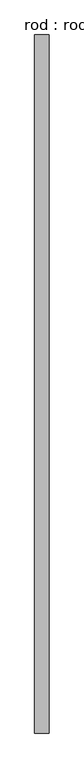
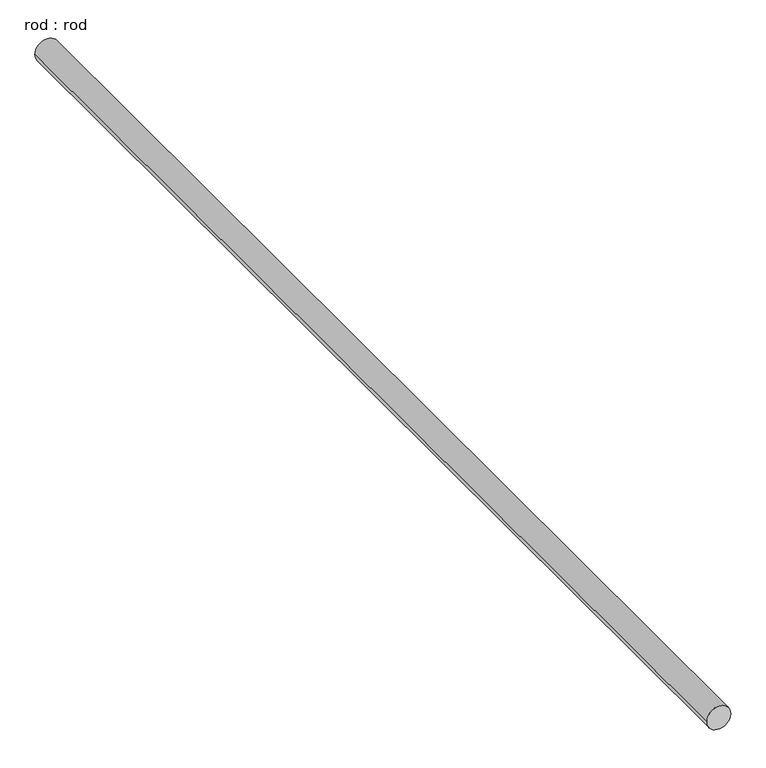
"""IFC4 building model written with IfcOpenShell, lengths in millimetres: proxy geometry, rod : rod."""

import ifcopenshell
import ifcopenshell.guid

model = None  # the IFC model being written
_history = None  # IfcOwnerHistory: only IFC2X3 demands one
_inside = {}  # id of a spatial element -> (the spatial element, [elements in it])
_under = {}  # id of a project, library or spatial element -> (it, [spatial elements below it])
_declared = {}  # id of a project -> (the project, [libraries it declares])
_typed = {}  # id of a type object -> (the type object, [elements of that type])
_made_of = {}  # id of a material, layer set ... -> (it, [elements and type objects made of it])


def new_model(schema):
    """Start an empty IFC model of exactly this schema.

    Asked for "IFC4X3", IfcOpenShell would pick the latest addendum, in which some entities
    have other attributes; the version numbers below select the first issue.
    IFC2X3 requires an IfcOwnerHistory on every rooted entity: one is made here for all.
    """
    global model, _history
    if schema == "IFC4X3":
        model = ifcopenshell.file(schema_version=(4, 3, 0, 0))
    else:
        model = ifcopenshell.file(schema=schema)
    _inside.clear()
    _under.clear()
    _declared.clear()
    _typed.clear()
    _made_of.clear()
    _history = None
    if model.schema == "IFC2X3":
        org = make("IfcOrganization", Name="unknown")
        user = make(
            "IfcPersonAndOrganization",
            ThePerson=make("IfcPerson", FamilyName="unknown"),
            TheOrganization=org,
        )
        app = make(
            "IfcApplication",
            ApplicationDeveloper=org,
            Version="unknown",
            ApplicationFullName="unknown",
            ApplicationIdentifier="unknown",
        )
        _history = make(
            "IfcOwnerHistory",
            OwningUser=user,
            OwningApplication=app,
            ChangeAction="ADDED",
            CreationDate=0,
        )
    return model


def make(cls, **values):
    """One entity of the class cls with the attributes given. An attribute that is None is left unset."""
    return model.create_entity(
        cls, **{name: value for name, value in values.items() if value is not None}
    )


def rooted(cls, **values):
    """An entity with a GlobalId (a new one), such as an element, a storey or a relation."""
    return make(cls, GlobalId=ifcopenshell.guid.new(), OwnerHistory=_history, **values)


def si_unit(unit_type, name, prefix=None):
    """IfcSIUnit, for example si_unit("LENGTHUNIT", "METRE", prefix="MILLI")."""
    return make("IfcSIUnit", UnitType=unit_type, Prefix=prefix, Name=name)


def assignment(units):
    """IfcUnitAssignment: the units of a project."""
    return None if units is None else make("IfcUnitAssignment", Units=units)


def point(xyz):
    """IfcCartesianPoint."""
    return None if xyz is None else make("IfcCartesianPoint", Coordinates=xyz)


def direction(xyz):
    """IfcDirection."""
    return None if xyz is None else make("IfcDirection", DirectionRatios=xyz)


def frame(location, z_axis=None, x_axis=None):
    """IfcAxis2Placement3D, a coordinate frame: its origin and axes. An axis left out is left unset."""
    return make(
        "IfcAxis2Placement3D",
        Location=point(location),
        Axis=direction(z_axis),
        RefDirection=direction(x_axis),
    )


def frame_2d(location, x_axis=None):
    """IfcAxis2Placement2D, a coordinate frame in the plane: its origin and x axis."""
    return make(
        "IfcAxis2Placement2D", Location=point(location), RefDirection=direction(x_axis)
    )


def origin():
    """The frame at (0, 0, 0) with its axes left unset."""
    return frame((0.0, 0.0, 0.0))


def place(relative_to, where):
    """IfcLocalPlacement: puts the frame where relative to a parent placement (None: the world)."""
    return make(
        "IfcLocalPlacement", PlacementRelTo=relative_to, RelativePlacement=where
    )


def context(
    kind, dimensions, precision=None, world=None, true_north=None, identifier=None
):
    """IfcGeometricRepresentationContext, for example the 3D "Model" context."""
    return make(
        "IfcGeometricRepresentationContext",
        ContextIdentifier=identifier,
        ContextType=kind,
        CoordinateSpaceDimension=dimensions,
        Precision=precision,
        WorldCoordinateSystem=world,
        TrueNorth=true_north,
    )


def project(units=None, contexts=None):
    """IfcProject with its units and contexts."""
    return rooted(
        "IfcProject",
        Name="project",
        RepresentationContexts=contexts,
        UnitsInContext=assignment(units),
    )


def spatial(cls, under=None, at=None, **own):
    """A site, building, storey or space (cls), placed at a placement, below another one or the project."""
    s = rooted(cls, ObjectPlacement=at, **own)
    if under is not None:
        _under.setdefault(under.id(), (under, []))[1].append(s)
    return s


def circle_curve(where, radius):
    """IfcCircle in the frame where."""
    return make("IfcCircle", Position=where, Radius=radius)


def trimmed(basis, trim1, trim2, sense, master):
    """IfcTrimmedCurve: the piece of a basis curve between two trims."""
    return make(
        "IfcTrimmedCurve",
        BasisCurve=basis,
        Trim1=trim1,
        Trim2=trim2,
        SenseAgreement=sense,
        MasterRepresentation=master,
    )


def segment(curve, same_sense, transition):
    """IfcCompositeCurveSegment."""
    return make(
        "IfcCompositeCurveSegment",
        Transition=transition,
        SameSense=same_sense,
        ParentCurve=curve,
    )


def composite_curve(segments, self_intersect=None):
    """IfcCompositeCurve: segments joined end to end."""
    return make("IfcCompositeCurve", Segments=segments, SelfIntersect=self_intersect)


def outline(outer, holes=None, kind="AREA"):
    """IfcArbitraryClosedProfileDef: a profile drawn as a closed curve; with holes, ...WithVoids."""
    if holes is None:
        return make("IfcArbitraryClosedProfileDef", ProfileType=kind, OuterCurve=outer)
    return make(
        "IfcArbitraryProfileDefWithVoids",
        ProfileType=kind,
        OuterCurve=outer,
        InnerCurves=holes,
    )


def extrude(swept, where, along, depth):
    """IfcExtrudedAreaSolid: the profile swept, set in the frame where, extruded along a direction by depth."""
    return make(
        "IfcExtrudedAreaSolid",
        SweptArea=swept,
        Position=where,
        ExtrudedDirection=direction(along),
        Depth=depth,
    )


def shape(context_of_items, identifier, shape_type, items):
    """IfcShapeRepresentation: the items that make up one representation, for example the "Body"."""
    return make(
        "IfcShapeRepresentation",
        ContextOfItems=context_of_items,
        RepresentationIdentifier=identifier,
        RepresentationType=shape_type,
        Items=items,
    )


def source(mapping_origin, context_of_items, identifier, shape_type, items):
    """IfcRepresentationMap: a shape defined once, which mapped items show again and again."""
    return make(
        "IfcRepresentationMap",
        MappingOrigin=mapping_origin,
        MappedRepresentation=shape(context_of_items, identifier, shape_type, items),
    )


def transform(
    local_origin,
    x_axis=None,
    y_axis=None,
    z_axis=None,
    scale=None,
    scale2=None,
    scale3=None,
    uniform=True,
):
    """IfcCartesianTransformationOperator3D, or its non-uniform kind. x_axis, y_axis, z_axis: its Axis1, 2, 3."""
    if uniform:
        return make(
            "IfcCartesianTransformationOperator3D",
            Axis1=direction(x_axis),
            Axis2=direction(y_axis),
            LocalOrigin=point(local_origin),
            Scale=scale,
            Axis3=direction(z_axis),
        )
    return make(
        "IfcCartesianTransformationOperator3DnonUniform",
        Axis1=direction(x_axis),
        Axis2=direction(y_axis),
        LocalOrigin=point(local_origin),
        Scale=scale,
        Axis3=direction(z_axis),
        Scale2=scale2,
        Scale3=scale3,
    )


def mapped(mapping_source, mapping_target):
    """IfcMappedItem: shows the shape of a source again, moved by a transform."""
    return make(
        "IfcMappedItem", MappingSource=mapping_source, MappingTarget=mapping_target
    )


def made_of(thing, what):
    """Note that an element or type object is made of a material, layer set ...; save() writes the relation."""
    if what is not None:
        _made_of.setdefault(what.id(), (what, []))[1].append(thing)
    return thing


def element(
    cls,
    number,
    at=None,
    inside=None,
    cuts=None,
    type_object=None,
    material=None,
    context=None,
    identifier="Body",
    shape_type=None,
    held_by="IfcProductDefinitionShape",
    body=None,
    shapes=None,
    **own,
):
    """One element of the class cls, such as IfcWall. Its Tag is "e" and its number.

    at: its placement. inside: the storey or other place that contains it. cuts: it is an
    opening in that element (IfcRelVoidsElement). A single representation is given by context,
    identifier, shape_type and body (its items); several are given by shapes. held_by: the class
    of the entity that holds the representations. save() writes the other relations.
    """
    e = rooted(cls, Tag="e%d" % number, ObjectPlacement=at, **own)
    if body is not None:
        shapes = [shape(context, identifier, shape_type, body)]
    if shapes is not None:
        e.Representation = make(held_by, Representations=shapes)
    if inside is not None:
        _inside.setdefault(inside.id(), (inside, []))[1].append(e)
    if cuts is not None:
        rooted(
            "IfcRelVoidsElement", RelatingBuildingElement=cuts, RelatedOpeningElement=e
        )
    if type_object is not None:
        _typed.setdefault(type_object.id(), (type_object, []))[1].append(e)
    return made_of(e, material)


def aggregate(whole, parts):
    """IfcRelAggregates: a whole, such as a stair, and the parts it consists of."""
    return rooted("IfcRelAggregates", RelatingObject=whole, RelatedObjects=parts)


def save(model, path):
    """Write the relations noted so far, then the file.

    IfcRelAggregates (storeys below a building ...), IfcRelContainedInSpatialStructure (elements
    in a storey), IfcRelDefinesByType, IfcRelAssociatesMaterial and IfcRelDeclares: one each for
    every whole, place, type object, material and project.
    """
    for whole, parts in _under.values():
        aggregate(whole, parts)
    for where, things in _inside.values():
        rooted(
            "IfcRelContainedInSpatialStructure",
            RelatedElements=things,
            RelatingStructure=where,
        )
    for kind, things in _typed.values():
        rooted("IfcRelDefinesByType", RelatedObjects=things, RelatingType=kind)
    for what, things in _made_of.values():
        rooted("IfcRelAssociatesMaterial", RelatedObjects=things, RelatingMaterial=what)
    for by, libraries in _declared.values():
        rooted("IfcRelDeclares", RelatingContext=by, RelatedDefinitions=libraries)
    model.write(path)


def rod_rod_e8d424b5(model_context):
    return source(origin(), model_context, "Body", "SweptSolid", [
        extrude(outline(composite_curve([segment(trimmed(circle_curve(frame_2d((0.0108462, 0.0)), 200.0), [point((0.0108462, 200.0))], [point((0.0108462, -200.0))], False, "CARTESIAN"), True, "CONTINUOUS"), segment(trimmed(circle_curve(frame_2d((0.0108462, 0.0)), 200.0), [point((0.0108462, -200.0))], [point((0.0108462, 200.0))], False, "CARTESIAN"), True, "CONTINUOUS")], self_intersect=False)), frame((0.0, -5502.5599022, 0.0), z_axis=(0.0, 1.0, 0.0), x_axis=(0.0, 0.0, 1.0)), (0.0, 0.0, 1.0), 19190.5770351),
    ])


if __name__ == "__main__":
    model = new_model("IFC4")
    model_context = context("Model", 3, world=origin())
    ifc_project = project(units=[si_unit("LENGTHUNIT", "METRE", prefix="MILLI")], contexts=[model_context])
    site = spatial("IfcSite", under=ifc_project)
    building = spatial("IfcBuilding", under=site)
    placement = place(None, origin())
    rod_rod_shape = rod_rod_e8d424b5(model_context)
    element("IfcBuildingElementProxy", 1, Name="rod : rod", ObjectType="rod : rod", at=placement, inside=building, context=model_context, shape_type="MappedRepresentation", body=[
        mapped(rod_rod_shape, transform((0.0, 0.0, 0.0), x_axis=(1.0, 0.0, 0.0), y_axis=(0.0, 1.0, 0.0), z_axis=(0.0, 0.0, 1.0))),
    ])
    save(model, "model.ifc")

# Revit data of these elements
# Type "rod : rod"
#   Default Elevation = 0
